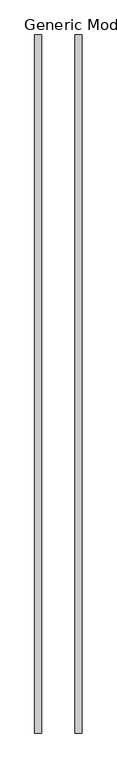
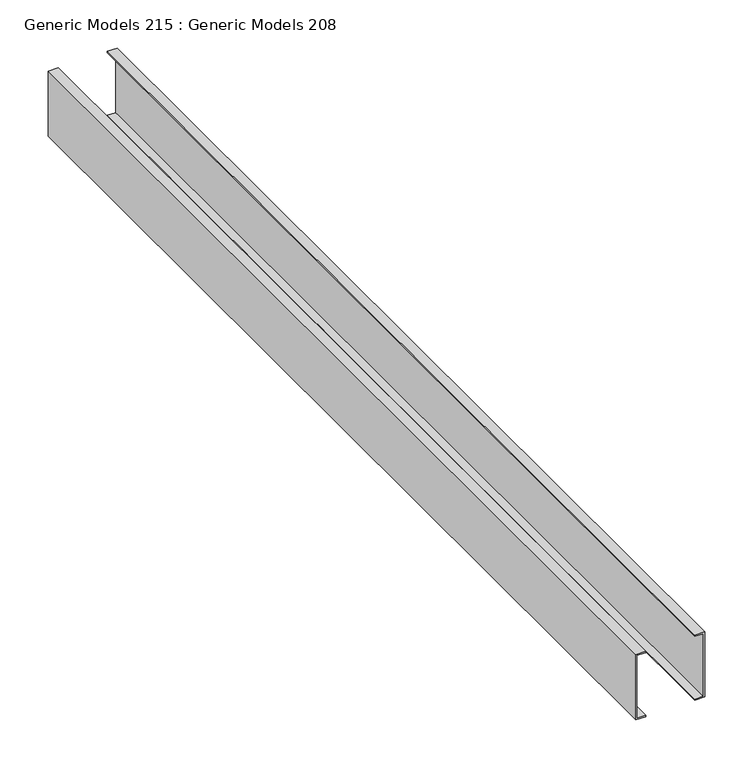
"""IFC4 building model written with IfcOpenShell, lengths in millimetres: proxy geometry, Generic Models 215 : Generic Models 208."""

from ifc_helpers import new_model, si_unit, frame, origin, place, context, project, spatial, polyline, outline, extrude, source, transform, mapped, element, save


def generic_models_215_generic_models_208_d85d510b(model_context):
    return source(origin(), model_context, "Body", "SweptSolid", [
        extrude(outline(polyline([(2257.425, 54459.9579676), (2257.425, 54448.1421489), (2255.8375, 54448.1421489), (2255.8375, 54458.3704676), (2176.4625, 54458.3704676), (2176.4625, 54448.1421489), (2174.875, 54448.1421489), (2174.875, 54459.9579676), (2257.425, 54459.9579676)])), frame((0.0, -228.7033818, 0.0), z_axis=(0.0, 1.0, 0.0), x_axis=(0.0, 0.0, 1.0)), (0.0, 0.0, 1.0), 1219.2),
        extrude(outline(polyline([(2257.425, 54377.4079676), (2174.875, 54377.4079676), (2174.875, 54389.2237864), (2176.4625, 54389.2237864), (2176.4625, 54378.9954676), (2255.8375, 54378.9954676), (2255.8375, 54389.2237864), (2257.425, 54389.2237864), (2257.425, 54377.4079676)])), frame((0.0, -228.7033818, 0.0), z_axis=(0.0, 1.0, 0.0), x_axis=(0.0, 0.0, 1.0)), (0.0, 0.0, 1.0), 1219.2),
    ])


if __name__ == "__main__":
    model = new_model("IFC4")
    model_context = context("Model", 3, world=origin())
    ifc_project = project(units=[si_unit("LENGTHUNIT", "METRE", prefix="MILLI")], contexts=[model_context])
    site = spatial("IfcSite", under=ifc_project)
    building = spatial("IfcBuilding", under=site)
    placement = place(None, origin())
    generic_models_215_generic_models_208_shape = generic_models_215_generic_models_208_d85d510b(model_context)
    element("IfcBuildingElementProxy", 1, Name="Generic Models 215 : Generic Models 208", ObjectType="Generic Models 215 : Generic Models 208", at=placement, inside=building, context=model_context, shape_type="MappedRepresentation", body=[
        mapped(generic_models_215_generic_models_208_shape, transform((0.0, 0.0, 0.0), x_axis=(1.0, 0.0, 0.0), y_axis=(0.0, 1.0, 0.0), z_axis=(0.0, 0.0, 1.0))),
    ])
    save(model, "model.ifc")
